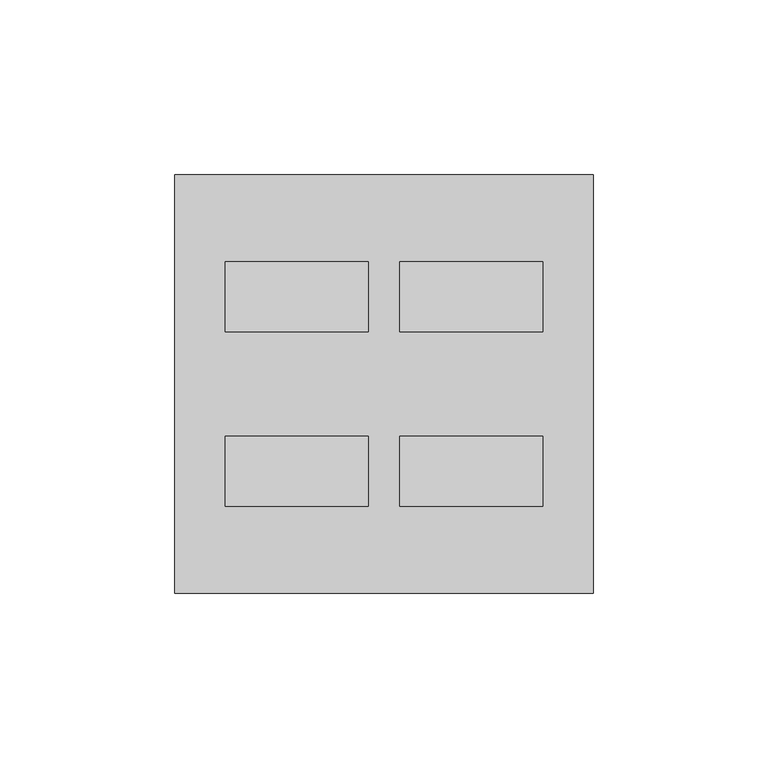
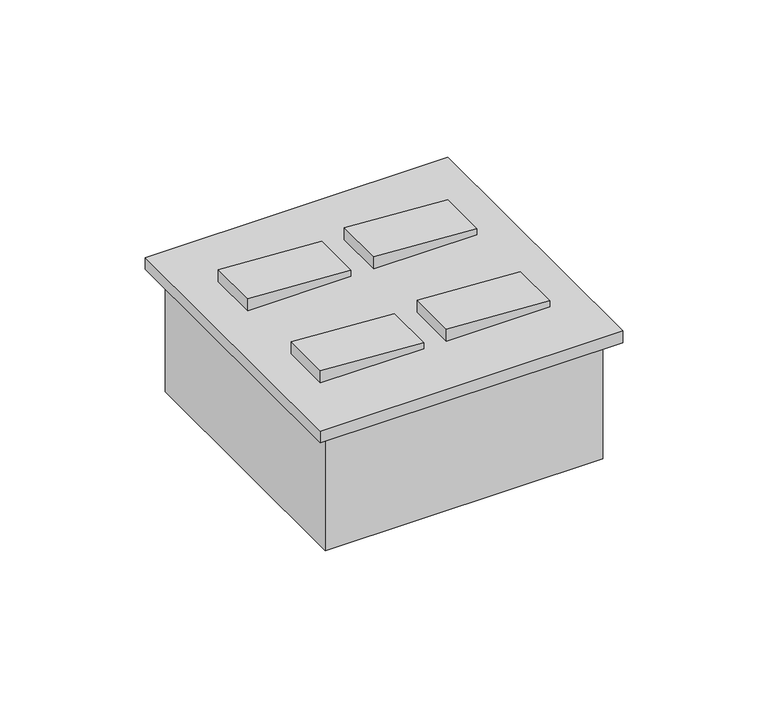
"""IFC4 building model written with IfcOpenShell, lengths in millimetres: proxy geometry, CAIXA VERTICE V7 : Interruptor 4s."""

from ifc_helpers import new_model, si_unit, frame, origin, origin_with_axes, place, context, project, spatial, polyline, outline, extrude, faceted_brep, source, transform, mapped, element, save


def electrical_fixtures_0cd0be00(model_context):
    return source(origin(), model_context, "Body", "SolidModel", [
        extrude(outline(polyline([(5.0, 45.5), (7.5, 45.5), (10.0, 4.5), (5.0, 4.5), (5.0, 45.5)])), frame((0.0, 1065.0, 0.0), z_axis=(0.0, 1.0, 0.0), x_axis=(0.0, 0.0, 1.0)), (0.0, 0.0, 1.0), 20.0),
        extrude(outline(polyline([(5.0, 45.5), (7.5, 45.5), (10.0, 4.5), (5.0, 4.5), (5.0, 45.5)])), frame((0.0, 1115.0, 0.0), z_axis=(0.0, 1.0, 0.0), x_axis=(0.0, 0.0, 1.0)), (0.0, 0.0, 1.0), 20.0),
        extrude(outline(polyline([(5.0, -4.5), (7.5, -4.5), (10.0, -45.5), (5.0, -45.5), (5.0, -4.5)])), frame((0.0, 1065.0, 0.0), z_axis=(0.0, 1.0, 0.0), x_axis=(0.0, 0.0, 1.0)), (0.0, 0.0, 1.0), 20.0),
        extrude(outline(polyline([(5.0, -4.5), (7.5, -4.5), (10.0, -45.5), (5.0, -45.5), (5.0, -4.5)])), frame((0.0, 1115.0, 0.0), z_axis=(0.0, 1.0, 0.0), x_axis=(0.0, 0.0, 1.0)), (0.0, 0.0, 1.0), 20.0),
        faceted_brep([(53.0, 1047.0, -48.0), (53.0, 1153.0, -48.0), (-53.0, 1153.0, -48.0), (-53.0, 1047.0, -48.0), (55.0, 1155.0, -50.0), (55.0, 1045.0, -50.0), (-55.0, 1045.0, -50.0), (-55.0, 1155.0, -50.0), (-55.0, 1155.0, 0.0), (55.0, 1155.0, 0.0), (-55.0, 1045.0, 0.0), (55.0, 1045.0, 0.0), (53.0, 1153.0, 0.0), (53.0, 1047.0, 0.0), (-53.0, 1047.0, 0.0), (-53.0, 1153.0, 0.0)], [[[0, 1, 2, 3]], [[4, 5, 6, 7]], [[4, 7, 8, 9]], [[8, 7, 6, 10]], [[10, 6, 5, 11]], [[11, 5, 4, 9]], [[9, 8, 10, 11], [12, 13, 14, 15]], [[13, 12, 1, 0]], [[14, 13, 0, 3]], [[15, 14, 3, 2]], [[12, 15, 2, 1]]]),
        extrude(outline(polyline([(60.0, 1160.0), (60.0, 1040.0), (-60.0, 1040.0), (-60.0, 1160.0), (60.0, 1160.0)])), origin_with_axes(), (0.0, 0.0, 1.0), 5.0),
    ])


if __name__ == "__main__":
    model = new_model("IFC4")
    model_context = context("Model", 3, world=origin())
    ifc_project = project(units=[si_unit("LENGTHUNIT", "METRE", prefix="MILLI")], contexts=[model_context])
    site = spatial("IfcSite", under=ifc_project)
    building = spatial("IfcBuilding", under=site)
    placement = place(None, origin())
    electrical_fixtures_shape = electrical_fixtures_0cd0be00(model_context)
    element("IfcBuildingElementProxy", 1, Name="CAIXA VERTICE V7 : Interruptor 4s", ObjectType="CAIXA VERTICE V7 : Interruptor 4s", at=placement, inside=building, context=model_context, shape_type="MappedRepresentation", body=[
        mapped(electrical_fixtures_shape, transform((0.0, 0.0, 0.0), x_axis=(1.0, 0.0, 0.0), y_axis=(0.0, 1.0, 0.0), z_axis=(0.0, 0.0, 1.0))),
    ])
    save(model, "model.ifc")

# Revit data of these elements
# Type "CAIXA VERTICE V7 : Interruptor 4s"
#   URL = "www.facebook.com/verticetreinamentos"
#   SEÇÃO [instance default] = ""
#   Rotação [instance default] = 0.00°
#   LARGURA DA TAMPA = 0.08 m
#   BORDA = 0.01 m
#   ALTURA DE INSTALAÇÃO [instance default] = 1.10 m
#   Distância Anotação [instance default] = 0.0015 m
#   ALTURA DA TAMPA = 0.12 m
#   Vertical [instance default] = yes
#   VER SEÇÃO [instance default] = yes
#   SHADE ESQ [instance default] = no
#   SHADE DIR [instance default] = yes
#   HORIZONTAL [instance default] = no
#   ANDAR COM A LEGENDA [instance default] = 0
#   Material Tampa [instance default] = Plástico, branco opaco
#   Caixa = element 1798512
#   Anotação = element 1798523
#   Default Elevation = 0
# Element 1 (IfcBuildingElementProxy, "CAIXA VERTICE V7 : Interruptor 4s")
#   SEÇÃO = "4"
#   Distância Anotação = 0.0035 m
#   ANDAR COM A LEGENDA = 1
#   Materials on its faces: "Plástico, branco opaco"
# Materials
#   "Plástico, branco opaco": class "Plástico", colour RGB 120 120 120, transparency 0, Description = "Plastic, generic, opaque white", Cost = 0
